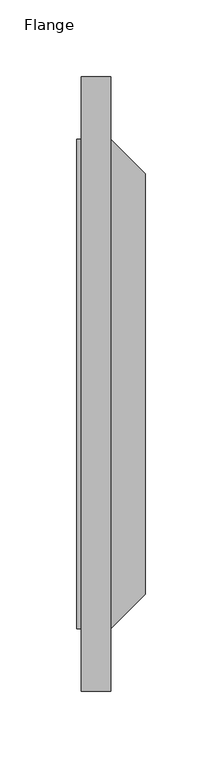
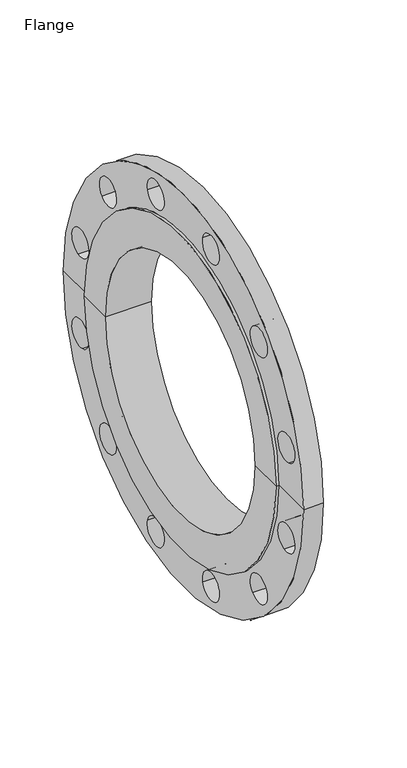
"""IFC4 building model written with IfcOpenShell, lengths in millimetres: proxy geometry, Flange : CASTED FLANGE PN16."""

from ifc_helpers import new_model, si_unit, frame, origin, place, context, project, spatial, polyline, circle_curve, source, transform, mapped, element, save
from ifc_brep_helpers import plane_surface, cylinder_surface, revolved_surface, advanced_brep


def flange_b74e5e12(model_context):
    return source(origin(), model_context, "Body", "AdvancedBrep", [
        advanced_brep(
        [(0.0, 125.0, 0.0), (0.0, 159.5, 0.0), (0.0, -159.5, 0.0), (0.0, -125.0, 0.0), (44.5, 125.0, 0.0), (44.5, -125.0, 0.0), (44.5, 137.0, 0.0), (44.5, -137.0, 0.0), (22.0, 159.5, 0.0), (22.0, -159.5, 0.0), (22.0, 200.0, 0.0), (22.0, -200.0, 0.0), (22.0, -59.4633421, -167.8283675), (22.0, -32.4174189, -175.0753008), (22.0, 32.4174189, -175.0753008), (22.0, 59.4633421, -167.8283675), (22.0, -135.4109486, -115.6119587), (22.0, -115.6119587, -135.4109486), (22.0, -175.0753008, -32.4174189), (22.0, -167.8283675, -59.4633421), (22.0, 167.8283675, -59.4633421), (22.0, 175.0753008, -32.4174189), (22.0, 115.6119587, -135.4109486), (22.0, 135.4109486, -115.6119587), (22.0, -32.4174189, 175.0753008), (22.0, -59.4633421, 167.8283675), (22.0, 59.4633421, 167.8283675), (22.0, 32.4174189, 175.0753008), (22.0, -167.8283675, 59.4633421), (22.0, -175.0753008, 32.4174189), (22.0, -115.6119587, 135.4109486), (22.0, -135.4109486, 115.6119587), (22.0, 135.4109486, 115.6119587), (22.0, 115.6119587, 135.4109486), (22.0, 175.0753008, 32.4174189), (22.0, 167.8283675, 59.4633421), (3.0, 200.0, 0.0), (3.0, -200.0, 0.0), (3.0, 159.5, 0.0), (3.0, -159.5, 0.0), (3.0, -32.4174189, -175.0753008), (3.0, -59.4633421, -167.8283675), (3.0, 59.4633421, -167.8283675), (3.0, 32.4174189, -175.0753008), (3.0, -115.6119587, -135.4109486), (3.0, -135.4109486, -115.6119587), (3.0, -167.8283675, -59.4633421), (3.0, -175.0753008, -32.4174189), (3.0, 175.0753008, -32.4174189), (3.0, 167.8283675, -59.4633421), (3.0, 135.4109486, -115.6119587), (3.0, 115.6119587, -135.4109486), (3.0, -59.4633421, 167.8283675), (3.0, -32.4174189, 175.0753008), (3.0, 32.4174189, 175.0753008), (3.0, 59.4633421, 167.8283675), (3.0, -175.0753008, 32.4174189), (3.0, -167.8283675, 59.4633421), (3.0, -135.4109486, 115.6119587), (3.0, -115.6119587, 135.4109486), (3.0, 115.6119587, 135.4109486), (3.0, 135.4109486, 115.6119587), (3.0, 167.8283675, 59.4633421), (3.0, 175.0753008, 32.4174189)],
        [
            (0, 1),
            (1, 2, circle_curve(frame((0.0, 0.0, 0.0), z_axis=(-1.0, 0.0, 0.0), x_axis=(0.0, 1.0, 0.0)), 159.5)),
            (2, 3),
            (3, 0, circle_curve(frame((0.0, 0.0, 0.0), z_axis=(1.0, 0.0, 0.0), x_axis=(0.0, 1.0, 0.0)), 125.0)),
            (0, 3, circle_curve(frame((0.0, 0.0, 0.0), z_axis=(1.0, 0.0, 0.0), x_axis=(0.0, 1.0, 0.0)), 125.0)),
            (2, 1, circle_curve(frame((0.0, 0.0, 0.0), z_axis=(-1.0, 0.0, 0.0), x_axis=(0.0, 1.0, 0.0)), 159.5)),
            (4, 0),
            (3, 5),
            (5, 4, circle_curve(frame((44.5, 0.0, 0.0), z_axis=(1.0, 0.0, 0.0), x_axis=(0.0, 1.0, 0.0)), 125.0)),
            (4, 5, circle_curve(frame((44.5, 0.0, 0.0), z_axis=(1.0, 0.0, 0.0), x_axis=(0.0, 1.0, 0.0)), 125.0)),
            (6, 4),
            (5, 7),
            (7, 6, circle_curve(frame((44.5, 0.0, 0.0), z_axis=(1.0, 0.0, 0.0), x_axis=(0.0, 1.0, 0.0)), 137.0)),
            (6, 7, circle_curve(frame((44.5, 0.0, 0.0), z_axis=(1.0, 0.0, 0.0), x_axis=(0.0, 1.0, 0.0)), 137.0)),
            (8, 6),
            (7, 9),
            (9, 8, circle_curve(frame((22.0, 0.0, 0.0), z_axis=(1.0, 0.0, 0.0), x_axis=(0.0, 1.0, 0.0)), 159.5)),
            (8, 9, circle_curve(frame((22.0, 0.0, 0.0), z_axis=(1.0, 0.0, 0.0), x_axis=(0.0, 1.0, 0.0)), 159.5)),
            (10, 8),
            (9, 11),
            (11, 10, circle_curve(frame((22.0, 0.0, 0.0), z_axis=(1.0, 0.0, 0.0), x_axis=(0.0, 1.0, 0.0)), 200.0)),
            (12, 13, circle_curve(frame((22.0, -45.9403805, -171.4518342), z_axis=(-1.0, 0.0, 0.0), x_axis=(0.0, 0.9659258262890734, -0.258819045102502)), 14.0)),
            (13, 12, circle_curve(frame((22.0, -45.9403805, -171.4518342), z_axis=(-1.0, 0.0, 0.0), x_axis=(0.0, 0.9659258262890734, -0.258819045102502)), 14.0)),
            (14, 15, circle_curve(frame((22.0, 45.9403805, -171.4518342), z_axis=(-1.0, 0.0, 0.0), x_axis=(0.0, 0.9659258262890654, 0.25881904510253184)), 14.0)),
            (15, 14, circle_curve(frame((22.0, 45.9403805, -171.4518342), z_axis=(-1.0, 0.0, 0.0), x_axis=(0.0, 0.9659258262890654, 0.25881904510253184)), 14.0)),
            (16, 17, circle_curve(frame((22.0, -125.5114537, -125.5114537), z_axis=(-1.0, 0.0, 0.0), x_axis=(0.0, 0.7071067811865748, -0.7071067811865202)), 14.0)),
            (17, 16, circle_curve(frame((22.0, -125.5114537, -125.5114537), z_axis=(-1.0, 0.0, 0.0), x_axis=(0.0, 0.7071067811865748, -0.7071067811865202)), 14.0)),
            (18, 19, circle_curve(frame((22.0, -171.4518342, -45.9403805), z_axis=(-1.0, 0.0, 0.0), x_axis=(0.0, 0.25881904510254733, -0.9659258262890613)), 14.0)),
            (19, 18, circle_curve(frame((22.0, -171.4518342, -45.9403805), z_axis=(-1.0, 0.0, 0.0), x_axis=(0.0, 0.25881904510254733, -0.9659258262890613)), 14.0)),
            (20, 21, circle_curve(frame((22.0, 171.4518342, -45.9403805), z_axis=(-1.0, 0.0, 0.0), x_axis=(0.0, 0.2588190451024855, 0.9659258262890777)), 14.0)),
            (21, 20, circle_curve(frame((22.0, 171.4518342, -45.9403805), z_axis=(-1.0, 0.0, 0.0), x_axis=(0.0, 0.2588190451024855, 0.9659258262890777)), 14.0)),
            (22, 23, circle_curve(frame((22.0, 125.5114537, -125.5114537), z_axis=(-1.0, 0.0, 0.0), x_axis=(0.0, 0.7071067811865215, 0.7071067811865739)), 14.0)),
            (23, 22, circle_curve(frame((22.0, 125.5114537, -125.5114537), z_axis=(-1.0, 0.0, 0.0), x_axis=(0.0, 0.7071067811865215, 0.7071067811865739)), 14.0)),
            (10, 11, circle_curve(frame((22.0, 0.0, 0.0), z_axis=(1.0, 0.0, 0.0), x_axis=(0.0, 1.0, 0.0)), 200.0)),
            (24, 25, circle_curve(frame((22.0, -45.9403805, 171.4518342), z_axis=(-1.0, 0.0, 0.0), x_axis=(0.0, -0.9659258262890627, -0.258819045102542)), 14.0)),
            (25, 24, circle_curve(frame((22.0, -45.9403805, 171.4518342), z_axis=(-1.0, 0.0, 0.0), x_axis=(0.0, -0.9659258262890627, -0.258819045102542)), 14.0)),
            (26, 27, circle_curve(frame((22.0, 45.9403805, 171.4518342), z_axis=(-1.0, 0.0, 0.0), x_axis=(0.0, -0.9659258262890742, 0.25881904510249887)), 14.0)),
            (27, 26, circle_curve(frame((22.0, 45.9403805, 171.4518342), z_axis=(-1.0, 0.0, 0.0), x_axis=(0.0, -0.9659258262890742, 0.25881904510249887)), 14.0)),
            (28, 29, circle_curve(frame((22.0, -171.4518342, 45.9403805), z_axis=(-1.0, 0.0, 0.0), x_axis=(0.0, -0.25881904510250014, -0.9659258262890739)), 14.0)),
            (29, 28, circle_curve(frame((22.0, -171.4518342, 45.9403805), z_axis=(-1.0, 0.0, 0.0), x_axis=(0.0, -0.25881904510250014, -0.9659258262890739)), 14.0)),
            (30, 31, circle_curve(frame((22.0, -125.5114537, 125.5114537), z_axis=(-1.0, 0.0, 0.0), x_axis=(0.0, -0.7071067811865321, -0.7071067811865631)), 14.0)),
            (31, 30, circle_curve(frame((22.0, -125.5114537, 125.5114537), z_axis=(-1.0, 0.0, 0.0), x_axis=(0.0, -0.7071067811865321, -0.7071067811865631)), 14.0)),
            (32, 33, circle_curve(frame((22.0, 125.5114537, 125.5114537), z_axis=(-1.0, 0.0, 0.0), x_axis=(0.0, -0.7071067811865728, 0.7071067811865224)), 14.0)),
            (33, 32, circle_curve(frame((22.0, 125.5114537, 125.5114537), z_axis=(-1.0, 0.0, 0.0), x_axis=(0.0, -0.7071067811865728, 0.7071067811865224)), 14.0)),
            (34, 35, circle_curve(frame((22.0, 171.4518342, 45.9403805), z_axis=(-1.0, 0.0, 0.0), x_axis=(0.0, -0.25881904510255627, 0.9659258262890589)), 14.0)),
            (35, 34, circle_curve(frame((22.0, 171.4518342, 45.9403805), z_axis=(-1.0, 0.0, 0.0), x_axis=(0.0, -0.25881904510255627, 0.9659258262890589)), 14.0)),
            (36, 10),
            (11, 37),
            (37, 36, circle_curve(frame((3.0, 0.0, 0.0), z_axis=(1.0, 0.0, 0.0), x_axis=(0.0, 1.0, 0.0)), 200.0)),
            (36, 37, circle_curve(frame((3.0, 0.0, 0.0), z_axis=(1.0, 0.0, 0.0), x_axis=(0.0, 1.0, 0.0)), 200.0)),
            (38, 36),
            (37, 39),
            (39, 38, circle_curve(frame((3.0, 0.0, 0.0), z_axis=(1.0, 0.0, 0.0), x_axis=(0.0, 1.0, 0.0)), 159.5)),
            (40, 41, circle_curve(frame((3.0, -45.9403805, -171.4518342), z_axis=(1.0, 0.0, 0.0), x_axis=(0.0, 0.9659258262890734, -0.258819045102502)), 14.0)),
            (41, 40, circle_curve(frame((3.0, -45.9403805, -171.4518342), z_axis=(1.0, 0.0, 0.0), x_axis=(0.0, 0.9659258262890734, -0.258819045102502)), 14.0)),
            (42, 43, circle_curve(frame((3.0, 45.9403805, -171.4518342), z_axis=(1.0, 0.0, 0.0), x_axis=(0.0, 0.9659258262890654, 0.25881904510253184)), 14.0)),
            (43, 42, circle_curve(frame((3.0, 45.9403805, -171.4518342), z_axis=(1.0, 0.0, 0.0), x_axis=(0.0, 0.9659258262890654, 0.25881904510253184)), 14.0)),
            (44, 45, circle_curve(frame((3.0, -125.5114537, -125.5114537), z_axis=(1.0, 0.0, 0.0), x_axis=(0.0, 0.7071067811865748, -0.7071067811865202)), 14.0)),
            (45, 44, circle_curve(frame((3.0, -125.5114537, -125.5114537), z_axis=(1.0, 0.0, 0.0), x_axis=(0.0, 0.7071067811865748, -0.7071067811865202)), 14.0)),
            (46, 47, circle_curve(frame((3.0, -171.4518342, -45.9403805), z_axis=(1.0, 0.0, 0.0), x_axis=(0.0, 0.25881904510254733, -0.9659258262890613)), 14.0)),
            (47, 46, circle_curve(frame((3.0, -171.4518342, -45.9403805), z_axis=(1.0, 0.0, 0.0), x_axis=(0.0, 0.25881904510254733, -0.9659258262890613)), 14.0)),
            (48, 49, circle_curve(frame((3.0, 171.4518342, -45.9403805), z_axis=(1.0, 0.0, 0.0), x_axis=(0.0, 0.2588190451024855, 0.9659258262890777)), 14.0)),
            (49, 48, circle_curve(frame((3.0, 171.4518342, -45.9403805), z_axis=(1.0, 0.0, 0.0), x_axis=(0.0, 0.2588190451024855, 0.9659258262890777)), 14.0)),
            (50, 51, circle_curve(frame((3.0, 125.5114537, -125.5114537), z_axis=(1.0, 0.0, 0.0), x_axis=(0.0, 0.7071067811865215, 0.7071067811865739)), 14.0)),
            (51, 50, circle_curve(frame((3.0, 125.5114537, -125.5114537), z_axis=(1.0, 0.0, 0.0), x_axis=(0.0, 0.7071067811865215, 0.7071067811865739)), 14.0)),
            (38, 39, circle_curve(frame((3.0, 0.0, 0.0), z_axis=(1.0, 0.0, 0.0), x_axis=(0.0, 1.0, 0.0)), 159.5)),
            (52, 53, circle_curve(frame((3.0, -45.9403805, 171.4518342), z_axis=(1.0, 0.0, 0.0), x_axis=(0.0, -0.9659258262890627, -0.258819045102542)), 14.0)),
            (53, 52, circle_curve(frame((3.0, -45.9403805, 171.4518342), z_axis=(1.0, 0.0, 0.0), x_axis=(0.0, -0.9659258262890627, -0.258819045102542)), 14.0)),
            (54, 55, circle_curve(frame((3.0, 45.9403805, 171.4518342), z_axis=(1.0, 0.0, 0.0), x_axis=(0.0, -0.9659258262890742, 0.25881904510249887)), 14.0)),
            (55, 54, circle_curve(frame((3.0, 45.9403805, 171.4518342), z_axis=(1.0, 0.0, 0.0), x_axis=(0.0, -0.9659258262890742, 0.25881904510249887)), 14.0)),
            (56, 57, circle_curve(frame((3.0, -171.4518342, 45.9403805), z_axis=(1.0, 0.0, 0.0), x_axis=(0.0, -0.25881904510250014, -0.9659258262890739)), 14.0)),
            (57, 56, circle_curve(frame((3.0, -171.4518342, 45.9403805), z_axis=(1.0, 0.0, 0.0), x_axis=(0.0, -0.25881904510250014, -0.9659258262890739)), 14.0)),
            (58, 59, circle_curve(frame((3.0, -125.5114537, 125.5114537), z_axis=(1.0, 0.0, 0.0), x_axis=(0.0, -0.7071067811865321, -0.7071067811865631)), 14.0)),
            (59, 58, circle_curve(frame((3.0, -125.5114537, 125.5114537), z_axis=(1.0, 0.0, 0.0), x_axis=(0.0, -0.7071067811865321, -0.7071067811865631)), 14.0)),
            (60, 61, circle_curve(frame((3.0, 125.5114537, 125.5114537), z_axis=(1.0, 0.0, 0.0), x_axis=(0.0, -0.7071067811865728, 0.7071067811865224)), 14.0)),
            (61, 60, circle_curve(frame((3.0, 125.5114537, 125.5114537), z_axis=(1.0, 0.0, 0.0), x_axis=(0.0, -0.7071067811865728, 0.7071067811865224)), 14.0)),
            (62, 63, circle_curve(frame((3.0, 171.4518342, 45.9403805), z_axis=(1.0, 0.0, 0.0), x_axis=(0.0, -0.25881904510255627, 0.9659258262890589)), 14.0)),
            (63, 62, circle_curve(frame((3.0, 171.4518342, 45.9403805), z_axis=(1.0, 0.0, 0.0), x_axis=(0.0, -0.25881904510255627, 0.9659258262890589)), 14.0)),
            (1, 38),
            (39, 2),
            (12, 41),
            (40, 13),
            (14, 43),
            (42, 15),
            (16, 45),
            (44, 17),
            (18, 47),
            (46, 19),
            (28, 57),
            (56, 29),
            (30, 59),
            (58, 31),
            (24, 53),
            (52, 25),
            (26, 55),
            (54, 27),
            (32, 61),
            (60, 33),
            (34, 63),
            (62, 35),
            (20, 49),
            (48, 21),
            (22, 51),
            (50, 23),
        ],
        [
            plane_surface(frame((0.0, 0.0, 0.0), z_axis=(-1.0, 0.0, 0.0), x_axis=(0.0, 1.0, 0.0))),
            revolved_surface(polyline([(0.0, 125.0, 0.0), (44.5, 125.0, 0.0)]), (-95.0, 0.0, 0.0), (-1.0, 0.0, 0.0)),
            plane_surface(frame((44.5, 0.0, 0.0), z_axis=(1.0, 0.0, 0.0), x_axis=(0.0, 1.0, 0.0))),
            revolved_surface(polyline([(44.5, 137.0, 0.0), (22.0, 159.5, 0.0)]), (-95.0, 0.0, 0.0), (-1.0, 0.0, 0.0)),
            plane_surface(frame((22.0, 0.0, 0.0), z_axis=(1.0, 0.0, 0.0), x_axis=(0.0, 1.0, 0.0))),
            cylinder_surface(frame((-95.0, 0.0, 0.0), z_axis=(-1.0, 0.0, 0.0), x_axis=(0.0, 1.0, 0.0)), 200.0),
            plane_surface(frame((3.0, 0.0, 0.0), z_axis=(-1.0, 0.0, 0.0), x_axis=(0.0, 1.0, 0.0))),
            cylinder_surface(frame((-95.0, 0.0, 0.0), z_axis=(-1.0, 0.0, 0.0), x_axis=(0.0, 1.0, 0.0)), 159.5),
            revolved_surface(polyline([(3.0, -32.41741893195297, -175.07530083143504), (22.0, -32.41741893195297, -175.07530083143504)]), (22.0, -45.9403805, -171.4518342), (-1.0, 0.0, 0.0)),
            revolved_surface(polyline([(3.0, 59.46334206804692, -167.82836756856457), (22.0, 59.46334206804692, -167.82836756856457)]), (22.0, 45.9403805, -171.4518342), (-1.0, 0.0, 0.0)),
            revolved_surface(polyline([(3.000000000000007, -115.61195876338796, -135.4109486366113), (22.0, -115.61195876338796, -135.4109486366113)]), (22.0, -125.5114537, -125.5114537), (-0.9999999999999998, 0.0, 0.0)),
            revolved_surface(polyline([(2.999999999999993, -167.82836756856435, -59.46334206804686), (22.0, -167.82836756856435, -59.46334206804686)]), (22.0, -171.4518342, -45.9403805), (-1.0000000000000002, 0.0, 0.0)),
            revolved_surface(polyline([(3.0, -175.07530083143502, 32.417418931952966), (22.0, -175.07530083143502, 32.417418931952966)]), (22.0, -171.4518342, 45.9403805), (-1.0, 0.0, 0.0)),
            revolved_surface(polyline([(3.0, -135.41094863661147, 115.61195876338812), (22.0, -135.41094863661147, 115.61195876338812)]), (22.0, -125.5114537, 125.5114537), (-1.0, 0.0, 0.0)),
            revolved_surface(polyline([(3.0, -59.463342068046884, 167.82836756856443), (22.0, -59.463342068046884, 167.82836756856443)]), (22.0, -45.9403805, 171.4518342), (-1.0, 0.0, 0.0)),
            revolved_surface(polyline([(3.0, 32.417418931952966, 175.075300831435), (22.0, 32.417418931952966, 175.075300831435)]), (22.0, 45.9403805, 171.4518342), (-1.0, 0.0, 0.0)),
            revolved_surface(polyline([(3.0, 115.61195876338799, 135.41094863661132), (22.0, 115.61195876338799, 135.41094863661132)]), (22.0, 125.5114537, 125.5114537), (-1.0, 0.0, 0.0)),
            revolved_surface(polyline([(3.0, 167.82836756856423, 59.46334206804683), (22.0, 167.82836756856423, 59.46334206804683)]), (22.0, 171.4518342, 45.9403805), (-1.0, 0.0, 0.0)),
            revolved_surface(polyline([(3.0, 175.07530083143482, -32.417418931952916), (22.0, 175.07530083143482, -32.417418931952916)]), (22.0, 171.4518342, -45.9403805), (-1.0, 0.0, 0.0)),
            revolved_surface(polyline([(2.999999999999993, 135.4109486366113, -115.61195876338797), (22.0, 135.4109486366113, -115.61195876338797)]), (22.0, 125.5114537, -125.5114537), (-1.0000000000000002, 0.0, 0.0)),
        ],
        [
            (0, [[1, 2, 3, 4]]),
            (0, [[-1, 5, -3, 6]]),
            (1, [[7, -4, 8, 9]]),
            (1, [[-7, 10, -8, -5]]),
            (2, [[11, -9, 12, 13]]),
            (2, [[-11, 14, -12, -10]]),
            (3, [[15, -13, 16, 17]]),
            (3, [[-15, 18, -16, -14]]),
            (4, [[19, -17, 20, 21], [22, 23], [24, 25], [26, 27], [28, 29], [30, 31], [32, 33]]),
            (4, [[-19, 34, -20, -18], [35, 36], [37, 38], [39, 40], [41, 42], [43, 44], [45, 46]]),
            (5, [[47, -21, 48, 49]]),
            (5, [[-47, 50, -48, -34]]),
            (6, [[51, -49, 52, 53], [54, 55], [56, 57], [58, 59], [60, 61], [62, 63], [64, 65]]),
            (6, [[-51, 66, -52, -50], [67, 68], [69, 70], [71, 72], [73, 74], [75, 76], [77, 78]]),
            (7, [[79, -53, 80, -2]]),
            (7, [[-79, -6, -80, -66]]),
            (8, [[81, -54, 82, -22]]),
            (8, [[-81, -23, -82, -55]]),
            (9, [[83, -56, 84, -24]]),
            (9, [[-83, -25, -84, -57]]),
            (10, [[85, -58, 86, -26]]),
            (10, [[-85, -27, -86, -59]]),
            (11, [[87, -60, 88, -28]]),
            (11, [[-87, -29, -88, -61]]),
            (12, [[89, -71, 90, -39]]),
            (12, [[-89, -40, -90, -72]]),
            (13, [[91, -73, 92, -41]]),
            (13, [[-91, -42, -92, -74]]),
            (14, [[93, -67, 94, -35]]),
            (14, [[-93, -36, -94, -68]]),
            (15, [[95, -69, 96, -37]]),
            (15, [[-95, -38, -96, -70]]),
            (16, [[97, -75, 98, -43]]),
            (16, [[-97, -44, -98, -76]]),
            (17, [[99, -77, 100, -45]]),
            (17, [[-99, -46, -100, -78]]),
            (18, [[101, -62, 102, -30]]),
            (18, [[-101, -31, -102, -63]]),
            (19, [[103, -64, 104, -32]]),
            (19, [[-103, -33, -104, -65]]),
        ],
    ),
    ])


if __name__ == "__main__":
    model = new_model("IFC4")
    model_context = context("Model", 3, world=origin())
    ifc_project = project(units=[si_unit("LENGTHUNIT", "METRE", prefix="MILLI")], contexts=[model_context])
    site = spatial("IfcSite", under=ifc_project)
    building = spatial("IfcBuilding", under=site)
    placement = place(None, origin())
    flange_shape = flange_b74e5e12(model_context)
    element("IfcBuildingElementProxy", 1, Name="Flange : CASTED FLANGE PN16", ObjectType="Flange : CASTED FLANGE PN16", at=placement, inside=building, context=model_context, shape_type="MappedRepresentation", body=[
        mapped(flange_shape, transform((0.0, 0.0, 0.0), x_axis=(1.0, 0.0, 0.0), y_axis=(0.0, 1.0, 0.0), z_axis=(0.0, 0.0, 1.0))),
    ])
    save(model, "model.ifc")

# Revit data of these elements
# Type "Flange : CASTED FLANGE PN16"
#   TABLE_DIMENSIONS = "DIMENSIONS FIXED FLANGE"
#   Short Description = ""
#   Description = "FIXED FLANGE"
#   K [instance default] = 110 mm
#   HOLE DIAMETER [instance default] = 19 mm
#   D4 [instance default] = 84 mm
#   DRILL DIAMETER [instance default] = 110 mm
#   DN [instance default] = 40 mm
#   D2 [instance default] = 70 mm
#   D [instance default] = 150 mm
#   f [instance default] = 3 mm
#   b [instance default] = 16 mm
#   ANGLE [instance default] = 45.00°
#   a [instance default] = 19 mm
#   PN = 16
#   BOLTS NUMBER [instance default] = 4
#   MATERIAL [instance default] = none
#   COATING [instance default] = none
#   Default Elevation = 0
# Element 1 (IfcBuildingElementProxy, "Flange : CASTED FLANGE PN16")
#   K = 355 mm
#   HOLE DIAMETER = 28 mm
#   D4 = 319 mm
#   DRILL DIAMETER = 355 mm
#   DN = 250 mm
#   D2 = 274 mm
#   D = 400 mm
#   b = 19 mm
#   a = 22 mm
#   BOLTS NUMBER = 12
#   COATING = Not informed
#   Materials on its faces: "Not informed"
# Materials
#   "Not informed": class "Paint/Coating", colour RGB 0 56 123, transparency 0, Description = "Not Informed", Cost = 0
